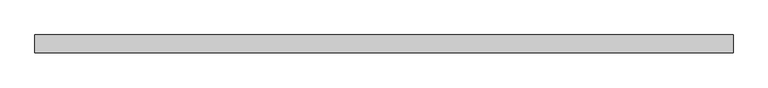
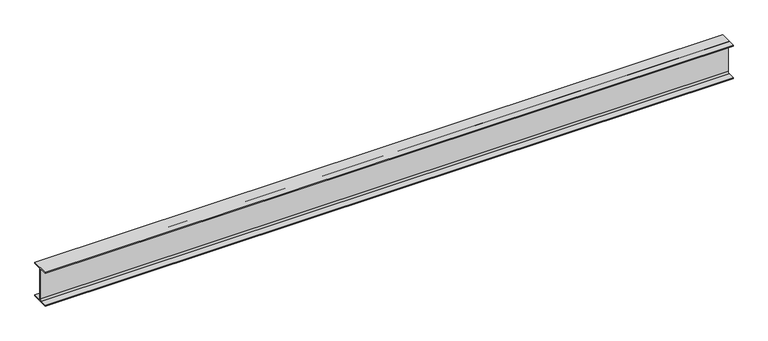
"""IFC4 building model written with IfcOpenShell, lengths in millimetres: beam geometry, Steel Framing_H_KS : H_SB_AR_S02_H-300x150x6.5x9_SRB3."""

import ifcopenshell
import ifcopenshell.guid

model = None  # the IFC model being written
_history = None  # IfcOwnerHistory: only IFC2X3 demands one
_inside = {}  # id of a spatial element -> (the spatial element, [elements in it])
_under = {}  # id of a project, library or spatial element -> (it, [spatial elements below it])
_declared = {}  # id of a project -> (the project, [libraries it declares])
_typed = {}  # id of a type object -> (the type object, [elements of that type])
_made_of = {}  # id of a material, layer set ... -> (it, [elements and type objects made of it])


def new_model(schema):
    """Start an empty IFC model of exactly this schema.

    Asked for "IFC4X3", IfcOpenShell would pick the latest addendum, in which some entities
    have other attributes; the version numbers below select the first issue.
    IFC2X3 requires an IfcOwnerHistory on every rooted entity: one is made here for all.
    """
    global model, _history
    if schema == "IFC4X3":
        model = ifcopenshell.file(schema_version=(4, 3, 0, 0))
    else:
        model = ifcopenshell.file(schema=schema)
    _inside.clear()
    _under.clear()
    _declared.clear()
    _typed.clear()
    _made_of.clear()
    _history = None
    if model.schema == "IFC2X3":
        org = make("IfcOrganization", Name="unknown")
        user = make(
            "IfcPersonAndOrganization",
            ThePerson=make("IfcPerson", FamilyName="unknown"),
            TheOrganization=org,
        )
        app = make(
            "IfcApplication",
            ApplicationDeveloper=org,
            Version="unknown",
            ApplicationFullName="unknown",
            ApplicationIdentifier="unknown",
        )
        _history = make(
            "IfcOwnerHistory",
            OwningUser=user,
            OwningApplication=app,
            ChangeAction="ADDED",
            CreationDate=0,
        )
    return model


def make(cls, **values):
    """One entity of the class cls with the attributes given. An attribute that is None is left unset."""
    return model.create_entity(
        cls, **{name: value for name, value in values.items() if value is not None}
    )


def rooted(cls, **values):
    """An entity with a GlobalId (a new one), such as an element, a storey or a relation."""
    return make(cls, GlobalId=ifcopenshell.guid.new(), OwnerHistory=_history, **values)


def si_unit(unit_type, name, prefix=None):
    """IfcSIUnit, for example si_unit("LENGTHUNIT", "METRE", prefix="MILLI")."""
    return make("IfcSIUnit", UnitType=unit_type, Prefix=prefix, Name=name)


def assignment(units):
    """IfcUnitAssignment: the units of a project."""
    return None if units is None else make("IfcUnitAssignment", Units=units)


def point(xyz):
    """IfcCartesianPoint."""
    return None if xyz is None else make("IfcCartesianPoint", Coordinates=xyz)


def direction(xyz):
    """IfcDirection."""
    return None if xyz is None else make("IfcDirection", DirectionRatios=xyz)


def frame(location, z_axis=None, x_axis=None):
    """IfcAxis2Placement3D, a coordinate frame: its origin and axes. An axis left out is left unset."""
    return make(
        "IfcAxis2Placement3D",
        Location=point(location),
        Axis=direction(z_axis),
        RefDirection=direction(x_axis),
    )


def frame_2d(location, x_axis=None):
    """IfcAxis2Placement2D, a coordinate frame in the plane: its origin and x axis."""
    return make(
        "IfcAxis2Placement2D", Location=point(location), RefDirection=direction(x_axis)
    )


def origin():
    """The frame at (0, 0, 0) with its axes left unset."""
    return frame((0.0, 0.0, 0.0))


def place(relative_to, where):
    """IfcLocalPlacement: puts the frame where relative to a parent placement (None: the world)."""
    return make(
        "IfcLocalPlacement", PlacementRelTo=relative_to, RelativePlacement=where
    )


def context(
    kind, dimensions, precision=None, world=None, true_north=None, identifier=None
):
    """IfcGeometricRepresentationContext, for example the 3D "Model" context."""
    return make(
        "IfcGeometricRepresentationContext",
        ContextIdentifier=identifier,
        ContextType=kind,
        CoordinateSpaceDimension=dimensions,
        Precision=precision,
        WorldCoordinateSystem=world,
        TrueNorth=true_north,
    )


def project(units=None, contexts=None):
    """IfcProject with its units and contexts."""
    return rooted(
        "IfcProject",
        Name="project",
        RepresentationContexts=contexts,
        UnitsInContext=assignment(units),
    )


def spatial(cls, under=None, at=None, **own):
    """A site, building, storey or space (cls), placed at a placement, below another one or the project."""
    s = rooted(cls, ObjectPlacement=at, **own)
    if under is not None:
        _under.setdefault(under.id(), (under, []))[1].append(s)
    return s


def polyline(points):
    """IfcPolyline through the points."""
    return make("IfcPolyline", Points=[point(p) for p in points])


def circle_curve(where, radius):
    """IfcCircle in the frame where."""
    return make("IfcCircle", Position=where, Radius=radius)


def trimmed(basis, trim1, trim2, sense, master):
    """IfcTrimmedCurve: the piece of a basis curve between two trims."""
    return make(
        "IfcTrimmedCurve",
        BasisCurve=basis,
        Trim1=trim1,
        Trim2=trim2,
        SenseAgreement=sense,
        MasterRepresentation=master,
    )


def segment(curve, same_sense, transition):
    """IfcCompositeCurveSegment."""
    return make(
        "IfcCompositeCurveSegment",
        Transition=transition,
        SameSense=same_sense,
        ParentCurve=curve,
    )


def composite_curve(segments, self_intersect=None):
    """IfcCompositeCurve: segments joined end to end."""
    return make("IfcCompositeCurve", Segments=segments, SelfIntersect=self_intersect)


def outline(outer, holes=None, kind="AREA"):
    """IfcArbitraryClosedProfileDef: a profile drawn as a closed curve; with holes, ...WithVoids."""
    if holes is None:
        return make("IfcArbitraryClosedProfileDef", ProfileType=kind, OuterCurve=outer)
    return make(
        "IfcArbitraryProfileDefWithVoids",
        ProfileType=kind,
        OuterCurve=outer,
        InnerCurves=holes,
    )


def extrude(swept, where, along, depth):
    """IfcExtrudedAreaSolid: the profile swept, set in the frame where, extruded along a direction by depth."""
    return make(
        "IfcExtrudedAreaSolid",
        SweptArea=swept,
        Position=where,
        ExtrudedDirection=direction(along),
        Depth=depth,
    )


def shape(context_of_items, identifier, shape_type, items):
    """IfcShapeRepresentation: the items that make up one representation, for example the "Body"."""
    return make(
        "IfcShapeRepresentation",
        ContextOfItems=context_of_items,
        RepresentationIdentifier=identifier,
        RepresentationType=shape_type,
        Items=items,
    )


def source(mapping_origin, context_of_items, identifier, shape_type, items):
    """IfcRepresentationMap: a shape defined once, which mapped items show again and again."""
    return make(
        "IfcRepresentationMap",
        MappingOrigin=mapping_origin,
        MappedRepresentation=shape(context_of_items, identifier, shape_type, items),
    )


def transform(
    local_origin,
    x_axis=None,
    y_axis=None,
    z_axis=None,
    scale=None,
    scale2=None,
    scale3=None,
    uniform=True,
):
    """IfcCartesianTransformationOperator3D, or its non-uniform kind. x_axis, y_axis, z_axis: its Axis1, 2, 3."""
    if uniform:
        return make(
            "IfcCartesianTransformationOperator3D",
            Axis1=direction(x_axis),
            Axis2=direction(y_axis),
            LocalOrigin=point(local_origin),
            Scale=scale,
            Axis3=direction(z_axis),
        )
    return make(
        "IfcCartesianTransformationOperator3DnonUniform",
        Axis1=direction(x_axis),
        Axis2=direction(y_axis),
        LocalOrigin=point(local_origin),
        Scale=scale,
        Axis3=direction(z_axis),
        Scale2=scale2,
        Scale3=scale3,
    )


def mapped(mapping_source, mapping_target):
    """IfcMappedItem: shows the shape of a source again, moved by a transform."""
    return make(
        "IfcMappedItem", MappingSource=mapping_source, MappingTarget=mapping_target
    )


def made_of(thing, what):
    """Note that an element or type object is made of a material, layer set ...; save() writes the relation."""
    if what is not None:
        _made_of.setdefault(what.id(), (what, []))[1].append(thing)
    return thing


def element(
    cls,
    number,
    at=None,
    inside=None,
    cuts=None,
    type_object=None,
    material=None,
    context=None,
    identifier="Body",
    shape_type=None,
    held_by="IfcProductDefinitionShape",
    body=None,
    shapes=None,
    **own,
):
    """One element of the class cls, such as IfcWall. Its Tag is "e" and its number.

    at: its placement. inside: the storey or other place that contains it. cuts: it is an
    opening in that element (IfcRelVoidsElement). A single representation is given by context,
    identifier, shape_type and body (its items); several are given by shapes. held_by: the class
    of the entity that holds the representations. save() writes the other relations.
    """
    e = rooted(cls, Tag="e%d" % number, ObjectPlacement=at, **own)
    if body is not None:
        shapes = [shape(context, identifier, shape_type, body)]
    if shapes is not None:
        e.Representation = make(held_by, Representations=shapes)
    if inside is not None:
        _inside.setdefault(inside.id(), (inside, []))[1].append(e)
    if cuts is not None:
        rooted(
            "IfcRelVoidsElement", RelatingBuildingElement=cuts, RelatedOpeningElement=e
        )
    if type_object is not None:
        _typed.setdefault(type_object.id(), (type_object, []))[1].append(e)
    return made_of(e, material)


def aggregate(whole, parts):
    """IfcRelAggregates: a whole, such as a stair, and the parts it consists of."""
    return rooted("IfcRelAggregates", RelatingObject=whole, RelatedObjects=parts)


def save(model, path):
    """Write the relations noted so far, then the file.

    IfcRelAggregates (storeys below a building ...), IfcRelContainedInSpatialStructure (elements
    in a storey), IfcRelDefinesByType, IfcRelAssociatesMaterial and IfcRelDeclares: one each for
    every whole, place, type object, material and project.
    """
    for whole, parts in _under.values():
        aggregate(whole, parts)
    for where, things in _inside.values():
        rooted(
            "IfcRelContainedInSpatialStructure",
            RelatedElements=things,
            RelatingStructure=where,
        )
    for kind, things in _typed.values():
        rooted("IfcRelDefinesByType", RelatedObjects=things, RelatingType=kind)
    for what, things in _made_of.values():
        rooted("IfcRelAssociatesMaterial", RelatedObjects=things, RelatingMaterial=what)
    for by, libraries in _declared.values():
        rooted("IfcRelDeclares", RelatingContext=by, RelatedDefinitions=libraries)
    model.write(path)


def beam_dc88aff0(model_context):
    return source(origin(), model_context, "Body", "SweptSolid", [
        extrude(outline(composite_curve([segment(polyline([(75.0, -141.0), (75.0, -150.0), (-75.0, -150.0), (-75.0, -141.0), (-16.25, -141.0)]), True, "CONTINUOUS"), segment(trimmed(circle_curve(frame_2d((-16.25, -128.0)), 13.0), [point((-16.25, -141.0))], [point((-3.25, -128.0))], True, "CARTESIAN"), True, "CONTINUOUS"), segment(polyline([(-3.25, -128.0), (-3.25, 128.0)]), True, "CONTINUOUS"), segment(trimmed(circle_curve(frame_2d((-16.25, 128.0)), 13.0), [point((-3.25, 128.0))], [point((-16.25, 141.0))], True, "CARTESIAN"), True, "CONTINUOUS"), segment(polyline([(-16.25, 141.0), (-75.0, 141.0), (-75.0, 150.0), (75.0, 150.0), (75.0, 141.0), (16.25, 141.0)]), True, "CONTINUOUS"), segment(trimmed(circle_curve(frame_2d((16.25, 128.0)), 13.0), [point((16.25, 141.0))], [point((3.25, 128.0))], True, "CARTESIAN"), True, "CONTINUOUS"), segment(polyline([(3.25, 128.0), (3.25, -128.0)]), True, "CONTINUOUS"), segment(trimmed(circle_curve(frame_2d((16.25, -128.0)), 13.0), [point((3.25, -128.0))], [point((16.25, -141.0))], True, "CARTESIAN"), True, "CONTINUOUS"), segment(polyline([(16.25, -141.0), (75.0, -141.0)]), True, "CONTINUOUS")], self_intersect=False)), frame((-2912.3, 0.0, 0.0), z_axis=(1.0, 0.0, 0.0), x_axis=(0.0, 1.0, 0.0)), (0.0, 0.0, 1.0), 5799.6),
    ])


if __name__ == "__main__":
    model = new_model("IFC4")
    model_context = context("Model", 3, world=origin())
    ifc_project = project(units=[si_unit("LENGTHUNIT", "METRE", prefix="MILLI")], contexts=[model_context])
    site = spatial("IfcSite", under=ifc_project)
    building = spatial("IfcBuilding", under=site)
    placement = place(None, origin())
    beam_shape = beam_dc88aff0(model_context)
    element("IfcBeam", 1, ObjectType="Steel Framing_H_KS : H_SB_AR_S02_H-300x150x6.5x9_SRB3", at=placement, inside=building, context=model_context, shape_type="MappedRepresentation", body=[
        mapped(beam_shape, transform((0.0, 0.0, 0.0), x_axis=(1.0, 0.0, 0.0), y_axis=(0.0, 1.0, 0.0), z_axis=(0.0, 0.0, 1.0))),
    ])
    save(model, "model.ifc")

# Revit data of these elements
# Type "Steel Framing_H_KS : H_SB_AR_S02_H-300x150x6.5x9_SRB3"
#   Type Comments = "MAIN"
#   Type Mark = "SRB3"
#   H_SectionID = "H-300x150x6.5x9"
#   H_Ratio for Additional Steel Plate = 0.2
#   Width = 15.0 cm
#   Web Thickness = 0.65 cm
#   Web Fillet = 1.3 cm
#   Warping Constant = 107000.0 cm⁶
#   Torsional Moment of Inertia = 9.9539 cm⁴
#   Section Area = 46.78 cm²
#   Plastic Modulus weak axis = 105.0 cm³
#   Plastic Modulus strong axis = 542.0 cm³
#   Perimeter = 1.17 m²/m
#   Nominal Weight = 36.70 kgf/m
#   Moment of Inertia weak axis = 508.00 cm⁴
#   Moment of Inertia strong axis = 7210.00 cm⁴
#   Height = 30.0 cm
#   Flange Thickness = 0.9 cm
#   Elastic Modulus weak axis = 67.7 cm³
#   Elastic Modulus strong axis = 481.0 cm³
#   Centroid Vertical = 15.0 cm
#   Centroid Horizontal = 7.5 cm
#   Bolt Spacing = 8.89 cm
#   Length [instance default] = 1500 mm
#   Structural Material [instance default] = Steel, 45-345
#   Section Name Key = ""
#   Assembly Code = ""
# Element 1 (IfcBeam, "Steel Framing_H_KS : H_SB_AR_S02_H-300x150x6.5x9_SRB3")
#   Materials on its faces: "Steel, 45-345"
# Materials
#   "Steel, 45-345": class "Metal", colour RGB 189 187 185, transparency 0, Description = "Steel 345 MPa", Cost = 0
